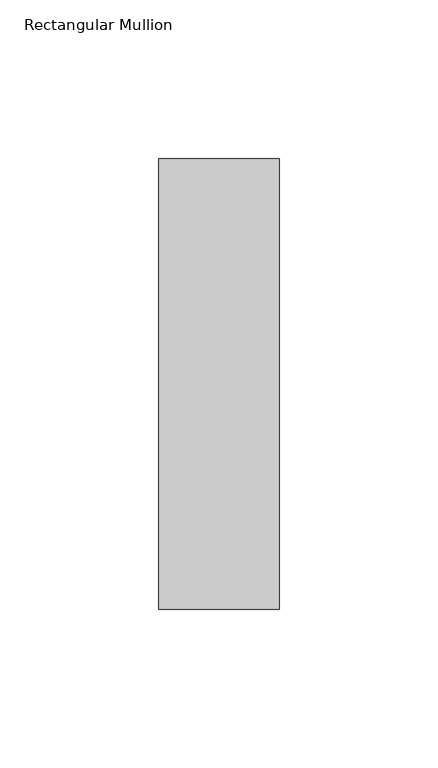
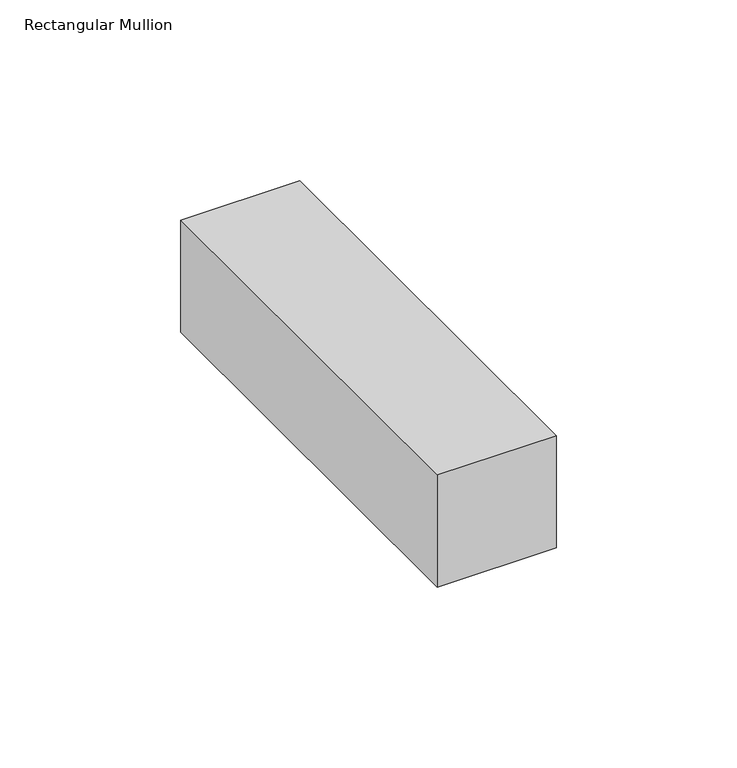
"""IFC4 building model written with IfcOpenShell, lengths in millimetres: member geometry, Rectangular Mullion : NLRS_21_CWM_hsb-regel 38x142_gen_rsf."""

import ifcopenshell
import ifcopenshell.guid

model = None  # the IFC model being written
_history = None  # IfcOwnerHistory: only IFC2X3 demands one
_inside = {}  # id of a spatial element -> (the spatial element, [elements in it])
_under = {}  # id of a project, library or spatial element -> (it, [spatial elements below it])
_declared = {}  # id of a project -> (the project, [libraries it declares])
_typed = {}  # id of a type object -> (the type object, [elements of that type])
_made_of = {}  # id of a material, layer set ... -> (it, [elements and type objects made of it])


def new_model(schema):
    """Start an empty IFC model of exactly this schema.

    Asked for "IFC4X3", IfcOpenShell would pick the latest addendum, in which some entities
    have other attributes; the version numbers below select the first issue.
    IFC2X3 requires an IfcOwnerHistory on every rooted entity: one is made here for all.
    """
    global model, _history
    if schema == "IFC4X3":
        model = ifcopenshell.file(schema_version=(4, 3, 0, 0))
    else:
        model = ifcopenshell.file(schema=schema)
    _inside.clear()
    _under.clear()
    _declared.clear()
    _typed.clear()
    _made_of.clear()
    _history = None
    if model.schema == "IFC2X3":
        org = make("IfcOrganization", Name="unknown")
        user = make(
            "IfcPersonAndOrganization",
            ThePerson=make("IfcPerson", FamilyName="unknown"),
            TheOrganization=org,
        )
        app = make(
            "IfcApplication",
            ApplicationDeveloper=org,
            Version="unknown",
            ApplicationFullName="unknown",
            ApplicationIdentifier="unknown",
        )
        _history = make(
            "IfcOwnerHistory",
            OwningUser=user,
            OwningApplication=app,
            ChangeAction="ADDED",
            CreationDate=0,
        )
    return model


def make(cls, **values):
    """One entity of the class cls with the attributes given. An attribute that is None is left unset."""
    return model.create_entity(
        cls, **{name: value for name, value in values.items() if value is not None}
    )


def rooted(cls, **values):
    """An entity with a GlobalId (a new one), such as an element, a storey or a relation."""
    return make(cls, GlobalId=ifcopenshell.guid.new(), OwnerHistory=_history, **values)


def si_unit(unit_type, name, prefix=None):
    """IfcSIUnit, for example si_unit("LENGTHUNIT", "METRE", prefix="MILLI")."""
    return make("IfcSIUnit", UnitType=unit_type, Prefix=prefix, Name=name)


def assignment(units):
    """IfcUnitAssignment: the units of a project."""
    return None if units is None else make("IfcUnitAssignment", Units=units)


def point(xyz):
    """IfcCartesianPoint."""
    return None if xyz is None else make("IfcCartesianPoint", Coordinates=xyz)


def direction(xyz):
    """IfcDirection."""
    return None if xyz is None else make("IfcDirection", DirectionRatios=xyz)


def frame(location, z_axis=None, x_axis=None):
    """IfcAxis2Placement3D, a coordinate frame: its origin and axes. An axis left out is left unset."""
    return make(
        "IfcAxis2Placement3D",
        Location=point(location),
        Axis=direction(z_axis),
        RefDirection=direction(x_axis),
    )


def origin():
    """The frame at (0, 0, 0) with its axes left unset."""
    return frame((0.0, 0.0, 0.0))


def place(relative_to, where):
    """IfcLocalPlacement: puts the frame where relative to a parent placement (None: the world)."""
    return make(
        "IfcLocalPlacement", PlacementRelTo=relative_to, RelativePlacement=where
    )


def context(
    kind, dimensions, precision=None, world=None, true_north=None, identifier=None
):
    """IfcGeometricRepresentationContext, for example the 3D "Model" context."""
    return make(
        "IfcGeometricRepresentationContext",
        ContextIdentifier=identifier,
        ContextType=kind,
        CoordinateSpaceDimension=dimensions,
        Precision=precision,
        WorldCoordinateSystem=world,
        TrueNorth=true_north,
    )


def project(units=None, contexts=None):
    """IfcProject with its units and contexts."""
    return rooted(
        "IfcProject",
        Name="project",
        RepresentationContexts=contexts,
        UnitsInContext=assignment(units),
    )


def spatial(cls, under=None, at=None, **own):
    """A site, building, storey or space (cls), placed at a placement, below another one or the project."""
    s = rooted(cls, ObjectPlacement=at, **own)
    if under is not None:
        _under.setdefault(under.id(), (under, []))[1].append(s)
    return s


def polyline(points):
    """IfcPolyline through the points."""
    return make("IfcPolyline", Points=[point(p) for p in points])


def outline(outer, holes=None, kind="AREA"):
    """IfcArbitraryClosedProfileDef: a profile drawn as a closed curve; with holes, ...WithVoids."""
    if holes is None:
        return make("IfcArbitraryClosedProfileDef", ProfileType=kind, OuterCurve=outer)
    return make(
        "IfcArbitraryProfileDefWithVoids",
        ProfileType=kind,
        OuterCurve=outer,
        InnerCurves=holes,
    )


def extrude(swept, where, along, depth):
    """IfcExtrudedAreaSolid: the profile swept, set in the frame where, extruded along a direction by depth."""
    return make(
        "IfcExtrudedAreaSolid",
        SweptArea=swept,
        Position=where,
        ExtrudedDirection=direction(along),
        Depth=depth,
    )


def shape(context_of_items, identifier, shape_type, items):
    """IfcShapeRepresentation: the items that make up one representation, for example the "Body"."""
    return make(
        "IfcShapeRepresentation",
        ContextOfItems=context_of_items,
        RepresentationIdentifier=identifier,
        RepresentationType=shape_type,
        Items=items,
    )


def source(mapping_origin, context_of_items, identifier, shape_type, items):
    """IfcRepresentationMap: a shape defined once, which mapped items show again and again."""
    return make(
        "IfcRepresentationMap",
        MappingOrigin=mapping_origin,
        MappedRepresentation=shape(context_of_items, identifier, shape_type, items),
    )


def transform(
    local_origin,
    x_axis=None,
    y_axis=None,
    z_axis=None,
    scale=None,
    scale2=None,
    scale3=None,
    uniform=True,
):
    """IfcCartesianTransformationOperator3D, or its non-uniform kind. x_axis, y_axis, z_axis: its Axis1, 2, 3."""
    if uniform:
        return make(
            "IfcCartesianTransformationOperator3D",
            Axis1=direction(x_axis),
            Axis2=direction(y_axis),
            LocalOrigin=point(local_origin),
            Scale=scale,
            Axis3=direction(z_axis),
        )
    return make(
        "IfcCartesianTransformationOperator3DnonUniform",
        Axis1=direction(x_axis),
        Axis2=direction(y_axis),
        LocalOrigin=point(local_origin),
        Scale=scale,
        Axis3=direction(z_axis),
        Scale2=scale2,
        Scale3=scale3,
    )


def mapped(mapping_source, mapping_target):
    """IfcMappedItem: shows the shape of a source again, moved by a transform."""
    return make(
        "IfcMappedItem", MappingSource=mapping_source, MappingTarget=mapping_target
    )


def made_of(thing, what):
    """Note that an element or type object is made of a material, layer set ...; save() writes the relation."""
    if what is not None:
        _made_of.setdefault(what.id(), (what, []))[1].append(thing)
    return thing


def element(
    cls,
    number,
    at=None,
    inside=None,
    cuts=None,
    type_object=None,
    material=None,
    context=None,
    identifier="Body",
    shape_type=None,
    held_by="IfcProductDefinitionShape",
    body=None,
    shapes=None,
    **own,
):
    """One element of the class cls, such as IfcWall. Its Tag is "e" and its number.

    at: its placement. inside: the storey or other place that contains it. cuts: it is an
    opening in that element (IfcRelVoidsElement). A single representation is given by context,
    identifier, shape_type and body (its items); several are given by shapes. held_by: the class
    of the entity that holds the representations. save() writes the other relations.
    """
    e = rooted(cls, Tag="e%d" % number, ObjectPlacement=at, **own)
    if body is not None:
        shapes = [shape(context, identifier, shape_type, body)]
    if shapes is not None:
        e.Representation = make(held_by, Representations=shapes)
    if inside is not None:
        _inside.setdefault(inside.id(), (inside, []))[1].append(e)
    if cuts is not None:
        rooted(
            "IfcRelVoidsElement", RelatingBuildingElement=cuts, RelatedOpeningElement=e
        )
    if type_object is not None:
        _typed.setdefault(type_object.id(), (type_object, []))[1].append(e)
    return made_of(e, material)


def aggregate(whole, parts):
    """IfcRelAggregates: a whole, such as a stair, and the parts it consists of."""
    return rooted("IfcRelAggregates", RelatingObject=whole, RelatedObjects=parts)


def save(model, path):
    """Write the relations noted so far, then the file.

    IfcRelAggregates (storeys below a building ...), IfcRelContainedInSpatialStructure (elements
    in a storey), IfcRelDefinesByType, IfcRelAssociatesMaterial and IfcRelDeclares: one each for
    every whole, place, type object, material and project.
    """
    for whole, parts in _under.values():
        aggregate(whole, parts)
    for where, things in _inside.values():
        rooted(
            "IfcRelContainedInSpatialStructure",
            RelatedElements=things,
            RelatingStructure=where,
        )
    for kind, things in _typed.values():
        rooted("IfcRelDefinesByType", RelatedObjects=things, RelatingType=kind)
    for what, things in _made_of.values():
        rooted("IfcRelAssociatesMaterial", RelatedObjects=things, RelatingMaterial=what)
    for by, libraries in _declared.values():
        rooted("IfcRelDeclares", RelatingContext=by, RelatedDefinitions=libraries)
    model.write(path)


def rectangular_mullion_c09c4bb1(model_context):
    return source(origin(), model_context, "Body", "SweptSolid", [
        extrude(outline(polyline([(19.0, -71.0), (-19.0, -71.0), (-19.0, 71.0), (19.0, 71.0), (19.0, -71.0)])), frame((0.0, 0.0, -38.0), z_axis=(0.0, 0.0, 1.0), x_axis=(1.0, 0.0, 0.0)), (0.0, 0.0, 1.0), 38.0),
    ])


if __name__ == "__main__":
    model = new_model("IFC4")
    model_context = context("Model", 3, world=origin())
    ifc_project = project(units=[si_unit("LENGTHUNIT", "METRE", prefix="MILLI")], contexts=[model_context])
    site = spatial("IfcSite", under=ifc_project)
    building = spatial("IfcBuilding", under=site)
    placement = place(None, origin())
    rectangular_mullion_shape = rectangular_mullion_c09c4bb1(model_context)
    element("IfcMember", 1, ObjectType="Rectangular Mullion : NLRS_21_CWM_hsb-regel 38x142_gen_rsf", at=placement, inside=building, context=model_context, shape_type="MappedRepresentation", body=[
        mapped(rectangular_mullion_shape, transform((0.0, 0.0, 0.0), x_axis=(1.0, 0.0, 0.0), y_axis=(0.0, 1.0, 0.0), z_axis=(0.0, 0.0, 1.0))),
    ])
    save(model, "model.ifc")

# Revit data of these elements
# Type "Rectangular Mullion : NLRS_21_CWM_hsb-regel 38x142_gen_rsf"
#   Export Type to IFC As = "IfcWall"
#   Type IfcGUID = "07M7mRoiH1CR8m_RSKIwpF"
#   Assembly Code = "21.10"
#   built-in parameter 1007322 = 0.465879 (stored number, unit not read)
#   built-in parameter 1007321 = 0.062336 (stored number, unit not read)
#   built-in parameter 1007320 = 0.062336 (stored number, unit not read)
# Element 1 (IfcMember, "Rectangular Mullion : NLRS_21_CWM_hsb-regel 38x142_gen_rsf")
#   Materials on its faces: "NLRS_i2_hout naaldhout vuren_gen_rsf"
# Materials
#   "NLRS_i2_hout naaldhout vuren_gen_rsf": class "I - Hout", colour RGB 234 199 147, transparency 0, Keynote = "i2", Manufacturer = "Revit Standards Foundation", URL = "www.revitstandards.org", Description = "hout vuren", Cost = 0
